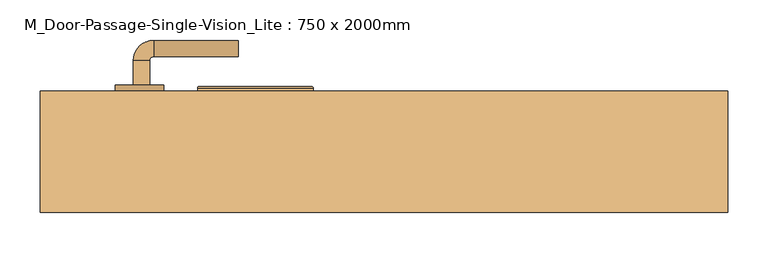
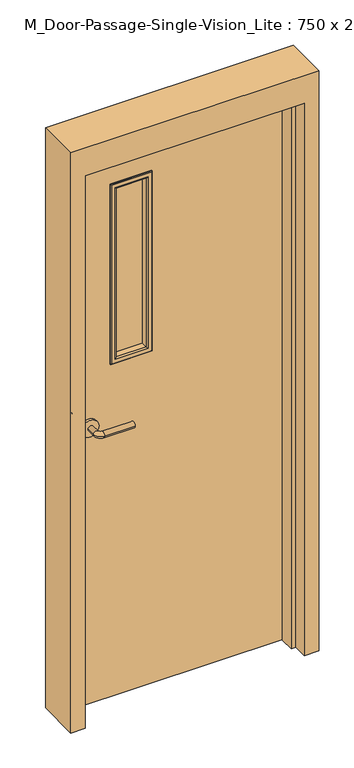
"""IFC4 building model written with IfcOpenShell, lengths in millimetres: door geometry, M_Door-Passage-Single-Vision_Lite : 750 x 2000mm."""

from ifc_helpers import new_model, si_unit, point, frame, frame_2d, origin, place, context, project, spatial, polyline, circle_curve, ellipse_curve, trimmed, segment, composite_curve, outline, extrude, faceted_brep, source, transform, mapped, element, save
from ifc_brep_helpers import plane_surface, cylinder_surface, revolved_surface, advanced_brep


def m_door_passage_single_vision_lite_750_x_2000mm_4b244377(model_context):
    return source(origin(), model_context, "Body", "SolidModel", [
        advanced_brep(
        [(-309.990625, 3.35, 1000.0), (-289.990625, 3.35, 1000.0), (-289.990625, -26.65, 1000.0), (-309.990625, -26.65, 1000.0), (-284.990625, -31.65, 1000.0), (-284.990625, -51.65, 1000.0), (-179.990625, -51.65, 1000.0), (-179.990625, -31.65, 1000.0)],
        [
            (0, 1, circle_curve(frame((-299.990625, 3.35, 1000.0), z_axis=(0.0, 1.0, 0.0), x_axis=(1.0, 0.0, 0.0)), 10.0)),
            (1, 0, circle_curve(frame((-299.990625, 3.35, 1000.0), z_axis=(0.0, 1.0, 0.0), x_axis=(1.0, 0.0, 0.0)), 10.0)),
            (1, 2),
            (2, 3, circle_curve(frame((-299.990625, -26.65, 1000.0), z_axis=(0.0, 1.0, 0.0), x_axis=(1.0, 0.0, 0.0)), 10.0)),
            (3, 0),
            (3, 2, circle_curve(frame((-299.990625, -26.65, 1000.0), z_axis=(0.0, 1.0, 0.0), x_axis=(1.0, 0.0, 0.0)), 10.0)),
            (4, 5, circle_curve(frame((-284.990625, -41.65, 1000.0), z_axis=(-1.0, 0.0, 0.0), x_axis=(0.0, 1.0, 0.0)), 10.0)),
            (5, 3, circle_curve(frame((-284.990625, -26.65, 1000.0), z_axis=(0.0, 0.0, -1.0), x_axis=(-1.0, 0.0, 0.0)), 25.0)),
            (2, 4, circle_curve(frame((-284.990625, -26.65, 1000.0), z_axis=(0.0, 0.0, 1.0), x_axis=(-1.0, 0.0, 0.0)), 5.0)),
            (5, 4, circle_curve(frame((-284.990625, -41.65, 1000.0), z_axis=(-1.0, 0.0, 0.0), x_axis=(0.0, 1.0, 0.0)), 10.0)),
            (6, 7, circle_curve(frame((-179.990625, -41.65, 1000.0), z_axis=(1.0, 0.0, 0.0), x_axis=(0.0, 1.0, 0.0)), 10.0)),
            (7, 6, circle_curve(frame((-179.990625, -41.65, 1000.0), z_axis=(1.0, 0.0, 0.0), x_axis=(0.0, 1.0, 0.0)), 10.0)),
            (4, 7),
            (6, 5),
        ],
        [
            plane_surface(frame((-299.990625, 3.35, 1000.0), z_axis=(0.0, 1.0, 0.0), x_axis=(0.0, 0.0, 1.0))),
            cylinder_surface(frame((-299.990625, 3.35, 1000.0), z_axis=(0.0, 1.0, 0.0), x_axis=(1.0, 0.0, 0.0)), 10.0),
            revolved_surface(trimmed(ellipse_curve(frame((-299.990625, -26.65, 1000.0), z_axis=(0.0, -1.0, 0.0), x_axis=(1.0, 0.0, 0.0)), 10.0, 10.0), [point((-309.990625, -26.65, 1000.0))], [point((-289.990625, -26.65, 1000.0))], True, "CARTESIAN"), (-284.990625, -26.65, 1000.0), (0.0, 0.0, -1.0)),
            revolved_surface(trimmed(ellipse_curve(frame((-299.990625, -26.65, 1000.0), z_axis=(0.0, -1.0, 0.0), x_axis=(1.0, 0.0, 0.0)), 10.0, 10.0), [point((-289.990625, -26.65, 1000.0))], [point((-309.990625, -26.65, 1000.0))], True, "CARTESIAN"), (-284.990625, -26.65, 1000.0), (0.0, 0.0, -1.0)),
            plane_surface(frame((-179.990625, -41.65, 1000.0), z_axis=(1.0, 0.0, 0.0), x_axis=(0.0, 0.0, 1.0))),
            cylinder_surface(frame((-284.990625, -41.65, 1000.0), z_axis=(-1.0, 0.0, 0.0), x_axis=(0.0, 1.0, 0.0)), 10.0),
        ],
        [
            (0, [[1, 2]]),
            (1, [[3, 4, 5, -2]]),
            (1, [[-5, 6, -3, -1]]),
            (2, [[7, 8, -4, 9]]),
            (3, [[10, -9, -6, -8]]),
            (4, [[11, 12]]),
            (5, [[13, -11, 14, -7]]),
            (5, [[-14, -12, -13, -10]]),
        ],
    ),
        extrude(outline(composite_curve([segment(trimmed(circle_curve(frame_2d((1000.0, -302.490625)), 30.0), [point((1000.0, -332.490625))], [point((1000.0, -272.490625))], False, "CARTESIAN"), True, "CONTINUOUS"), segment(trimmed(circle_curve(frame_2d((1000.0, -302.490625)), 30.0), [point((1000.0, -272.490625))], [point((1000.0, -332.490625))], False, "CARTESIAN"), True, "CONTINUOUS")], self_intersect=False)), frame((0.0, 3.35, 0.0), z_axis=(0.0, 1.0, 0.0), x_axis=(0.0, 0.0, 1.0)), (0.0, 0.0, 1.0), 8.0),
        advanced_brep(
        [(-309.990625, 64.35, 1000.0), (-289.990625, 64.35, 1000.0), (-309.990625, 94.35, 1000.0), (-289.990625, 94.35, 1000.0), (-284.990625, 99.35, 1000.0), (-284.990625, 119.35, 1000.0), (-179.990625, 119.35, 1000.0), (-179.990625, 99.35, 1000.0)],
        [
            (0, 1, circle_curve(frame((-299.990625, 64.35, 1000.0), z_axis=(0.0, -1.0, 0.0), x_axis=(1.0, 0.0, 0.0)), 10.0)),
            (1, 0, circle_curve(frame((-299.990625, 64.35, 1000.0), z_axis=(0.0, -1.0, 0.0), x_axis=(1.0, 0.0, 0.0)), 10.0)),
            (0, 2),
            (2, 3, circle_curve(frame((-299.990625, 94.35, 1000.0), z_axis=(0.0, -1.0, 0.0), x_axis=(1.0, 0.0, 0.0)), 10.0)),
            (3, 1),
            (3, 2, circle_curve(frame((-299.990625, 94.35, 1000.0), z_axis=(0.0, -1.0, 0.0), x_axis=(1.0, 0.0, 0.0)), 10.0)),
            (4, 3, circle_curve(frame((-284.990625, 94.35, 1000.0), z_axis=(0.0, 0.0, 1.0), x_axis=(-1.0, 0.0, 0.0)), 5.0)),
            (2, 5, circle_curve(frame((-284.990625, 94.35, 1000.0), z_axis=(0.0, 0.0, -1.0), x_axis=(-1.0, 0.0, 0.0)), 25.0)),
            (5, 4, circle_curve(frame((-284.990625, 109.35, 1000.0), z_axis=(-1.0, 0.0, 0.0), x_axis=(0.0, -1.0, 0.0)), 10.0)),
            (4, 5, circle_curve(frame((-284.990625, 109.35, 1000.0), z_axis=(-1.0, 0.0, 0.0), x_axis=(0.0, -1.0, 0.0)), 10.0)),
            (6, 7, circle_curve(frame((-179.990625, 109.35, 1000.0), z_axis=(1.0, 0.0, 0.0), x_axis=(0.0, -1.0, 0.0)), 10.0)),
            (7, 6, circle_curve(frame((-179.990625, 109.35, 1000.0), z_axis=(1.0, 0.0, 0.0), x_axis=(0.0, -1.0, 0.0)), 10.0)),
            (5, 6),
            (7, 4),
        ],
        [
            plane_surface(frame((-299.990625, 64.35, 1000.0), z_axis=(0.0, -1.0, 0.0), x_axis=(0.0, 0.0, 1.0))),
            cylinder_surface(frame((-299.990625, 64.35, 1000.0), z_axis=(0.0, -1.0, 0.0), x_axis=(1.0, 0.0, 0.0)), 10.0),
            revolved_surface(trimmed(ellipse_curve(frame((-299.990625, 94.35, 1000.0), z_axis=(0.0, -1.0, 0.0), x_axis=(1.0, 0.0, 0.0)), 10.0, 10.0), [point((-309.990625, 94.35, 1000.0))], [point((-289.990625, 94.35, 1000.0))], True, "CARTESIAN"), (-284.990625, 94.35, 1000.0), (0.0, 0.0, -1.0)),
            revolved_surface(trimmed(ellipse_curve(frame((-299.990625, 94.35, 1000.0), z_axis=(0.0, -1.0, 0.0), x_axis=(1.0, 0.0, 0.0)), 10.0, 10.0), [point((-289.990625, 94.35, 1000.0))], [point((-309.990625, 94.35, 1000.0))], True, "CARTESIAN"), (-284.990625, 94.35, 1000.0), (0.0, 0.0, -1.0)),
            plane_surface(frame((-179.990625, 109.35, 1000.0), z_axis=(1.0, 0.0, 0.0), x_axis=(0.0, 0.0, 1.0))),
            cylinder_surface(frame((-284.990625, 109.35, 1000.0), z_axis=(-1.0, 0.0, 0.0), x_axis=(0.0, -1.0, 0.0)), 10.0),
        ],
        [
            (0, [[1, 2]]),
            (1, [[-1, 3, 4, 5]]),
            (1, [[-2, -5, 6, -3]]),
            (2, [[7, -4, 8, 9]]),
            (3, [[-8, -6, -7, 10]]),
            (4, [[11, 12]]),
            (5, [[-9, 13, -12, 14]]),
            (5, [[-10, -14, -11, -13]]),
        ],
    ),
        extrude(outline(composite_curve([segment(trimmed(circle_curve(frame_2d((1000.0, -302.490625)), 30.0), [point((1000.0, -332.490625))], [point((1000.0, -272.490625))], False, "CARTESIAN"), True, "CONTINUOUS"), segment(trimmed(circle_curve(frame_2d((1000.0, -302.490625)), 30.0), [point((1000.0, -272.490625))], [point((1000.0, -332.490625))], False, "CARTESIAN"), True, "CONTINUOUS")], self_intersect=False)), frame((0.0, 56.35, 0.0), z_axis=(0.0, 1.0, 0.0), x_axis=(0.0, 0.0, 1.0)), (0.0, 0.0, 1.0), 8.0),
        extrude(outline(polyline([(2000.0, -375.0), (0.0, -375.0), (0.0, 375.0), (2000.0, 375.0), (2000.0, -375.0)]), holes=[polyline([(1847.6, -222.6), (1847.6, -95.6), (1212.6, -95.6), (1212.6, -222.6), (1847.6, -222.6)])]), frame((0.0, 11.35, 0.0), z_axis=(0.0, 1.0, 0.0), x_axis=(0.0, 0.0, 1.0)), (0.0, 0.0, 1.0), 45.0),
        faceted_brep([(375.0, 6.5875, 0.0), (375.0, 56.35, 0.0), (425.0, 56.35, 0.0), (425.0, -93.65, 0.0), (375.0, -93.65, 0.0), (375.0, -44.4375, 0.0), (359.125, -44.4375, 0.0), (359.125, 6.5875, 0.0), (375.0, 6.5875, 2000.0), (375.0, 56.35, 2000.0), (-375.0, 56.35, 2000.0), (-375.0, 56.35, 0.0), (-425.0, 56.35, 0.0), (-425.0, 56.35, 2100.0), (425.0, 56.35, 2100.0), (425.0, -93.65, 2100.0), (-425.0, -93.65, 2100.0), (-425.0, -93.65, 0.0), (-375.0, -93.65, 0.0), (-375.0, -93.65, 2000.0), (375.0, -93.65, 2000.0), (375.0, -44.4375, 2000.0), (-375.0, -44.4375, 2000.0), (-375.0, -44.4375, 0.0), (-359.125, -44.4375, 0.0), (-359.125, -44.4375, 1984.125), (359.125, -44.4375, 1984.125), (359.125, 6.5875, 1984.125), (-359.125, 6.5875, 1984.125), (-359.125, 6.5875, 0.0), (-375.0, 6.5875, 0.0), (-375.0, 6.5875, 2000.0)], [[[0, 1, 2, 3, 4, 5, 6, 7]], [[1, 0, 8, 9]], [[2, 1, 9, 10, 11, 12, 13, 14]], [[3, 2, 14, 15]], [[4, 3, 15, 16, 17, 18, 19, 20]], [[5, 4, 20, 21]], [[6, 5, 21, 22, 23, 24, 25, 26]], [[7, 6, 26, 27]], [[0, 7, 27, 28, 29, 30, 31, 8]], [[9, 8, 31, 10]], [[20, 19, 22, 21]], [[26, 25, 28, 27]], [[12, 11, 30, 29, 24, 23, 18, 17]], [[11, 10, 31, 30]], [[13, 12, 17, 16]], [[19, 18, 23, 22]], [[25, 24, 29, 28]], [[15, 14, 13, 16]]]),
        extrude(outline(polyline([(-95.6, 31.35), (-222.6, 31.35), (-222.6, 36.35), (-95.6, 36.35), (-95.6, 31.35)])), frame((0.0, 0.0, 1212.6), z_axis=(0.0, 0.0, 1.0), x_axis=(1.0, 0.0, 0.0)), (0.0, 0.0, 1.0), 635.0),
        advanced_brep(
        [(-222.6, 36.35, 1847.6), (-222.6, 56.35, 1847.6), (-222.6, 56.35, 1212.6), (-222.6, 36.35, 1212.6), (-210.6, 57.35, 1835.6), (-210.6, 36.35, 1835.6), (-210.6, 36.35, 1224.6), (-210.6, 57.35, 1224.6), (-215.6, 62.35, 1840.6), (-215.6, 62.35, 1219.6), (-230.6, 60.35, 1855.6), (-228.6, 62.35, 1853.6), (-228.6, 62.35, 1206.6), (-230.6, 60.35, 1204.6), (-230.6, 56.35, 1855.6), (-230.6, 56.35, 1204.6), (-95.6, 56.35, 1212.6), (-95.6, 36.35, 1212.6), (-107.6, 36.35, 1224.6), (-107.6, 57.35, 1224.6), (-102.6, 62.35, 1219.6), (-89.6, 62.35, 1206.6), (-87.6, 60.35, 1204.6), (-87.6, 56.35, 1204.6), (-95.6, 56.35, 1847.6), (-95.6, 36.35, 1847.6), (-107.6, 36.35, 1835.6), (-107.6, 57.35, 1835.6), (-102.6, 62.35, 1840.6), (-89.6, 62.35, 1853.6), (-87.6, 60.35, 1855.6), (-87.6, 56.35, 1855.6)],
        [
            (0, 1),
            (1, 2),
            (2, 3),
            (3, 0),
            (4, 5),
            (5, 6),
            (6, 7),
            (7, 4),
            (8, 4, ellipse_curve(frame((-215.6, 57.35, 1840.6), z_axis=(-0.7071067811865475, 0.0, -0.7071067811865475), x_axis=(-0.7071067811865474, 0.0, 0.7071067811865476)), 7.0710678, 5.0)),
            (7, 9, ellipse_curve(frame((-215.6, 57.35, 1219.6), z_axis=(-0.7071067811865475, 0.0, 0.7071067811865475), x_axis=(0.7071067811865474, 0.0, 0.7071067811865476)), 7.0710678, 5.0)),
            (9, 8),
            (10, 11, ellipse_curve(frame((-228.6, 60.35, 1853.6), z_axis=(-0.7071067811865475, 0.0, -0.7071067811865475), x_axis=(-0.7071067811865474, 0.0, 0.7071067811865476)), 2.8284271, 2.0)),
            (11, 12),
            (12, 13, ellipse_curve(frame((-228.6, 60.35, 1206.6), z_axis=(-0.7071067811865475, 0.0, 0.7071067811865475), x_axis=(0.7071067811865474, 0.0, 0.7071067811865476)), 2.8284271, 2.0)),
            (13, 10),
            (14, 10),
            (13, 15),
            (15, 14),
            (2, 16),
            (16, 17),
            (17, 3),
            (6, 18),
            (18, 19),
            (19, 7),
            (19, 20, ellipse_curve(frame((-102.6, 57.35, 1219.6), z_axis=(-0.7071067811865475, 0.0, -0.7071067811865475), x_axis=(-0.7071067811865476, 0.0, 0.7071067811865474)), 7.0710678, 5.0)),
            (20, 9),
            (12, 21),
            (21, 22, ellipse_curve(frame((-89.6, 60.35, 1206.6), z_axis=(-0.7071067811865475, 0.0, -0.7071067811865475), x_axis=(-0.7071067811865476, 0.0, 0.7071067811865474)), 2.8284271, 2.0)),
            (22, 13),
            (22, 23),
            (23, 15),
            (16, 24),
            (24, 25),
            (25, 17),
            (18, 26),
            (26, 27),
            (27, 19),
            (27, 28, ellipse_curve(frame((-102.6, 57.35, 1840.6), z_axis=(0.7071067811865475, 0.0, -0.7071067811865475), x_axis=(-0.7071067811865474, 0.0, -0.7071067811865476)), 7.0710678, 5.0)),
            (28, 20),
            (21, 29),
            (29, 30, ellipse_curve(frame((-89.6, 60.35, 1853.6), z_axis=(0.7071067811865475, 0.0, -0.7071067811865475), x_axis=(-0.7071067811865474, 0.0, -0.7071067811865476)), 2.8284271, 2.0)),
            (30, 22),
            (30, 31),
            (31, 23),
            (31, 14),
            (1, 24),
            (0, 25),
            (5, 26),
            (4, 27),
            (8, 28),
            (11, 29),
            (10, 30),
        ],
        [
            plane_surface(frame((-222.6, 56.35, 1847.6), z_axis=(-1.0, 0.0, 0.0), x_axis=(0.0, 0.0, -1.0))),
            plane_surface(frame((-210.6, 36.35, 1835.6), z_axis=(1.0, 0.0, 0.0), x_axis=(0.0, 0.0, -1.0))),
            cylinder_surface(frame((-215.6, 57.35, 1847.6), z_axis=(0.0, 0.0, 1.0), x_axis=(-1.0, 0.0, 0.0)), 5.0),
            cylinder_surface(frame((-228.6, 60.35, 1847.6), z_axis=(0.0, 0.0, 1.0), x_axis=(-1.0, 0.0, 0.0)), 2.0),
            plane_surface(frame((-230.6, 60.35, 1855.6), z_axis=(-1.0, 0.0, 0.0), x_axis=(0.0, 0.0, -1.0))),
            plane_surface(frame((-222.6, 56.35, 1212.6), z_axis=(0.0, 0.0, -1.0), x_axis=(1.0, 0.0, 0.0))),
            plane_surface(frame((-210.6, 36.35, 1224.6), z_axis=(0.0, 0.0, 1.0), x_axis=(1.0, 0.0, 0.0))),
            cylinder_surface(frame((-222.6, 57.35, 1219.6), z_axis=(-1.0, 0.0, 0.0), x_axis=(0.0, 0.0, -1.0)), 5.0),
            cylinder_surface(frame((-222.6, 60.35, 1206.6), z_axis=(-1.0, 0.0, 0.0), x_axis=(0.0, 0.0, -1.0)), 2.0),
            plane_surface(frame((-230.6, 60.35, 1204.6), z_axis=(0.0, 0.0, -1.0), x_axis=(1.0, 0.0, 0.0))),
            plane_surface(frame((-95.6, 56.35, 1212.6), z_axis=(1.0, 0.0, 0.0), x_axis=(0.0, 0.0, 1.0))),
            plane_surface(frame((-107.6, 36.35, 1224.6), z_axis=(-1.0, 0.0, 0.0), x_axis=(0.0, 0.0, 1.0))),
            cylinder_surface(frame((-102.6, 57.35, 1212.6), z_axis=(0.0, 0.0, -1.0), x_axis=(1.0, 0.0, 0.0)), 5.0),
            cylinder_surface(frame((-89.6, 60.35, 1212.6), z_axis=(0.0, 0.0, -1.0), x_axis=(1.0, 0.0, 0.0)), 2.0),
            plane_surface(frame((-87.6, 60.35, 1204.6), z_axis=(1.0, 0.0, 0.0), x_axis=(0.0, 0.0, 1.0))),
            plane_surface(frame((-87.6, 56.35, 1855.6), z_axis=(0.0, -1.0, 0.0), x_axis=(-1.0, 0.0, 0.0))),
            plane_surface(frame((-95.6, 56.35, 1847.6), z_axis=(0.0, 0.0, 1.0), x_axis=(-1.0, 0.0, 0.0))),
            plane_surface(frame((-95.6, 36.35, 1847.6), z_axis=(0.0, -1.0, 0.0), x_axis=(-1.0, 0.0, 0.0))),
            plane_surface(frame((-107.6, 36.35, 1835.6), z_axis=(0.0, 0.0, -1.0), x_axis=(-1.0, 0.0, 0.0))),
            cylinder_surface(frame((-95.6, 57.35, 1840.6), z_axis=(1.0, 0.0, 0.0), x_axis=(0.0, 0.0, 1.0)), 5.0),
            plane_surface(frame((-102.6, 62.35, 1840.6), z_axis=(0.0, 1.0, 0.0), x_axis=(-1.0, 0.0, 0.0))),
            cylinder_surface(frame((-95.6, 60.35, 1853.6), z_axis=(1.0, 0.0, 0.0), x_axis=(0.0, 0.0, 1.0)), 2.0),
            plane_surface(frame((-87.6, 60.35, 1855.6), z_axis=(0.0, 0.0, 1.0), x_axis=(-1.0, 0.0, 0.0))),
        ],
        [
            (0, [[1, 2, 3, 4]]),
            (1, [[5, 6, 7, 8]]),
            (2, [[9, -8, 10, 11]]),
            (3, [[12, 13, 14, 15]]),
            (4, [[16, -15, 17, 18]]),
            (5, [[-3, 19, 20, 21]]),
            (6, [[-7, 22, 23, 24]]),
            (7, [[-10, -24, 25, 26]]),
            (8, [[-14, 27, 28, 29]]),
            (9, [[-17, -29, 30, 31]]),
            (10, [[-20, 32, 33, 34]]),
            (11, [[-23, 35, 36, 37]]),
            (12, [[-25, -37, 38, 39]]),
            (13, [[-28, 40, 41, 42]]),
            (14, [[-30, -42, 43, 44]]),
            (15, [[-31, -44, 45, -18], [46, -32, -19, -2]]),
            (16, [[-33, -46, -1, 47]]),
            (17, [[-21, -34, -47, -4], [48, -35, -22, -6]]),
            (18, [[-36, -48, -5, 49]]),
            (19, [[-38, -49, -9, 50]]),
            (20, [[51, -40, -27, -13], [-26, -39, -50, -11]]),
            (21, [[-41, -51, -12, 52]]),
            (22, [[-43, -52, -16, -45]]),
        ],
    ),
        advanced_brep(
        [(-222.6, 31.35, 1212.6), (-222.6, 11.35, 1212.6), (-222.6, 11.35, 1847.6), (-222.6, 31.35, 1847.6), (-210.6, 10.35, 1224.6), (-210.6, 31.35, 1224.6), (-210.6, 31.35, 1835.6), (-210.6, 10.35, 1835.6), (-215.6, 5.35, 1219.6), (-215.6, 5.35, 1840.6), (-230.6, 7.35, 1204.6), (-228.6, 5.35, 1206.6), (-228.6, 5.35, 1853.6), (-230.6, 7.35, 1855.6), (-230.6, 11.35, 1204.6), (-230.6, 11.35, 1855.6), (-95.6, 11.35, 1847.6), (-95.6, 31.35, 1847.6), (-107.6, 31.35, 1835.6), (-107.6, 10.35, 1835.6), (-102.6, 5.35, 1840.6), (-89.6, 5.35, 1853.6), (-87.6, 7.35, 1855.6), (-87.6, 11.35, 1855.6), (-95.6, 11.35, 1212.6), (-95.6, 31.35, 1212.6), (-107.6, 31.35, 1224.6), (-107.6, 10.35, 1224.6), (-102.6, 5.35, 1219.6), (-89.6, 5.35, 1206.6), (-87.6, 7.35, 1204.6), (-87.6, 11.35, 1204.6)],
        [
            (0, 1),
            (1, 2),
            (2, 3),
            (3, 0),
            (4, 5),
            (5, 6),
            (6, 7),
            (7, 4),
            (8, 4, ellipse_curve(frame((-215.6, 10.35, 1219.6), z_axis=(-0.7071067811865475, 0.0, 0.7071067811865475), x_axis=(-0.7071067811865474, 0.0, -0.7071067811865476)), 7.0710678, 5.0)),
            (7, 9, ellipse_curve(frame((-215.6, 10.35, 1840.6), z_axis=(-0.7071067811865475, 0.0, -0.7071067811865475), x_axis=(0.7071067811865474, 0.0, -0.7071067811865476)), 7.0710678, 5.0)),
            (9, 8),
            (10, 11, ellipse_curve(frame((-228.6, 7.35, 1206.6), z_axis=(-0.7071067811865475, 0.0, 0.7071067811865475), x_axis=(-0.7071067811865474, 0.0, -0.7071067811865476)), 2.8284271, 2.0)),
            (11, 12),
            (12, 13, ellipse_curve(frame((-228.6, 7.35, 1853.6), z_axis=(-0.7071067811865475, 0.0, -0.7071067811865475), x_axis=(0.7071067811865474, 0.0, -0.7071067811865476)), 2.8284271, 2.0)),
            (13, 10),
            (14, 10),
            (13, 15),
            (15, 14),
            (2, 16),
            (16, 17),
            (17, 3),
            (6, 18),
            (18, 19),
            (19, 7),
            (19, 20, ellipse_curve(frame((-102.6, 10.35, 1840.6), z_axis=(-0.7071067811865475, 0.0, 0.7071067811865475), x_axis=(-0.7071067811865476, 0.0, -0.7071067811865474)), 7.0710678, 5.0)),
            (20, 9),
            (12, 21),
            (21, 22, ellipse_curve(frame((-89.6, 7.35, 1853.6), z_axis=(-0.7071067811865475, 0.0, 0.7071067811865475), x_axis=(-0.7071067811865476, 0.0, -0.7071067811865474)), 2.8284271, 2.0)),
            (22, 13),
            (22, 23),
            (23, 15),
            (16, 24),
            (24, 25),
            (25, 17),
            (18, 26),
            (26, 27),
            (27, 19),
            (27, 28, ellipse_curve(frame((-102.6, 10.35, 1219.6), z_axis=(0.7071067811865475, 0.0, 0.7071067811865475), x_axis=(-0.7071067811865474, 0.0, 0.7071067811865476)), 7.0710678, 5.0)),
            (28, 20),
            (21, 29),
            (29, 30, ellipse_curve(frame((-89.6, 7.35, 1206.6), z_axis=(0.7071067811865475, 0.0, 0.7071067811865475), x_axis=(-0.7071067811865474, 0.0, 0.7071067811865476)), 2.8284271, 2.0)),
            (30, 22),
            (30, 31),
            (31, 23),
            (31, 14),
            (1, 24),
            (0, 25),
            (5, 26),
            (4, 27),
            (8, 28),
            (11, 29),
            (10, 30),
        ],
        [
            plane_surface(frame((-222.6, 11.35, 1212.6), z_axis=(-1.0, 0.0, 0.0), x_axis=(0.0, 0.0, 1.0))),
            plane_surface(frame((-210.6, 31.35, 1224.6), z_axis=(1.0, 0.0, 0.0), x_axis=(0.0, 0.0, 1.0))),
            cylinder_surface(frame((-215.6, 10.35, 1212.6), z_axis=(0.0, 0.0, -1.0), x_axis=(-1.0, 0.0, 0.0)), 5.0),
            cylinder_surface(frame((-228.6, 7.35, 1212.6), z_axis=(0.0, 0.0, -1.0), x_axis=(-1.0, 0.0, 0.0)), 2.0),
            plane_surface(frame((-230.6, 7.35, 1204.6), z_axis=(-1.0, 0.0, 0.0), x_axis=(0.0, 0.0, 1.0))),
            plane_surface(frame((-222.6, 11.35, 1847.6), z_axis=(0.0, 0.0, 1.0), x_axis=(1.0, 0.0, 0.0))),
            plane_surface(frame((-210.6, 31.35, 1835.6), z_axis=(0.0, 0.0, -1.0), x_axis=(1.0, 0.0, 0.0))),
            cylinder_surface(frame((-222.6, 10.35, 1840.6), z_axis=(-1.0, 0.0, 0.0), x_axis=(0.0, 0.0, 1.0)), 5.0),
            cylinder_surface(frame((-222.6, 7.35, 1853.6), z_axis=(-1.0, 0.0, 0.0), x_axis=(0.0, 0.0, 1.0)), 2.0),
            plane_surface(frame((-230.6, 7.35, 1855.6), z_axis=(0.0, 0.0, 1.0), x_axis=(1.0, 0.0, 0.0))),
            plane_surface(frame((-95.6, 11.35, 1847.6), z_axis=(1.0, 0.0, 0.0), x_axis=(0.0, 0.0, -1.0))),
            plane_surface(frame((-107.6, 31.35, 1835.6), z_axis=(-1.0, 0.0, 0.0), x_axis=(0.0, 0.0, -1.0))),
            cylinder_surface(frame((-102.6, 10.35, 1847.6), z_axis=(0.0, 0.0, 1.0), x_axis=(1.0, 0.0, 0.0)), 5.0),
            cylinder_surface(frame((-89.6, 7.35, 1847.6), z_axis=(0.0, 0.0, 1.0), x_axis=(1.0, 0.0, 0.0)), 2.0),
            plane_surface(frame((-87.6, 7.35, 1855.6), z_axis=(1.0, 0.0, 0.0), x_axis=(0.0, 0.0, -1.0))),
            plane_surface(frame((-87.6, 11.35, 1204.6), z_axis=(0.0, 1.0, 0.0), x_axis=(-1.0, 0.0, 0.0))),
            plane_surface(frame((-95.6, 11.35, 1212.6), z_axis=(0.0, 0.0, -1.0), x_axis=(-1.0, 0.0, 0.0))),
            plane_surface(frame((-95.6, 31.35, 1212.6), z_axis=(0.0, 1.0, 0.0), x_axis=(-1.0, 0.0, 0.0))),
            plane_surface(frame((-107.6, 31.35, 1224.6), z_axis=(0.0, 0.0, 1.0), x_axis=(-1.0, 0.0, 0.0))),
            cylinder_surface(frame((-95.6, 10.35, 1219.6), z_axis=(1.0, 0.0, 0.0), x_axis=(0.0, 0.0, -1.0)), 5.0),
            plane_surface(frame((-102.6, 5.35, 1219.6), z_axis=(0.0, -1.0, 0.0), x_axis=(-1.0, 0.0, 0.0))),
            cylinder_surface(frame((-95.6, 7.35, 1206.6), z_axis=(1.0, 0.0, 0.0), x_axis=(0.0, 0.0, -1.0)), 2.0),
            plane_surface(frame((-87.6, 7.35, 1204.6), z_axis=(0.0, 0.0, -1.0), x_axis=(-1.0, 0.0, 0.0))),
        ],
        [
            (0, [[1, 2, 3, 4]]),
            (1, [[5, 6, 7, 8]]),
            (2, [[9, -8, 10, 11]]),
            (3, [[12, 13, 14, 15]]),
            (4, [[16, -15, 17, 18]]),
            (5, [[-3, 19, 20, 21]]),
            (6, [[-7, 22, 23, 24]]),
            (7, [[-10, -24, 25, 26]]),
            (8, [[-14, 27, 28, 29]]),
            (9, [[-17, -29, 30, 31]]),
            (10, [[-20, 32, 33, 34]]),
            (11, [[-23, 35, 36, 37]]),
            (12, [[-25, -37, 38, 39]]),
            (13, [[-28, 40, 41, 42]]),
            (14, [[-30, -42, 43, 44]]),
            (15, [[-31, -44, 45, -18], [46, -32, -19, -2]]),
            (16, [[-33, -46, -1, 47]]),
            (17, [[-21, -34, -47, -4], [48, -35, -22, -6]]),
            (18, [[-36, -48, -5, 49]]),
            (19, [[-38, -49, -9, 50]]),
            (20, [[51, -40, -27, -13], [-26, -39, -50, -11]]),
            (21, [[-41, -51, -12, 52]]),
            (22, [[-43, -52, -16, -45]]),
        ],
    ),
    ])


if __name__ == "__main__":
    model = new_model("IFC4")
    model_context = context("Model", 3, world=origin())
    ifc_project = project(units=[si_unit("LENGTHUNIT", "METRE", prefix="MILLI")], contexts=[model_context])
    site = spatial("IfcSite", under=ifc_project)
    building = spatial("IfcBuilding", under=site)
    placement = place(None, origin())
    m_door_passage_single_vision_lite_750_x_2000mm_shape = m_door_passage_single_vision_lite_750_x_2000mm_4b244377(model_context)
    element("IfcDoor", 1, ObjectType="M_Door-Passage-Single-Vision_Lite : 750 x 2000mm", at=placement, inside=building, context=model_context, shape_type="MappedRepresentation", body=[
        mapped(m_door_passage_single_vision_lite_750_x_2000mm_shape, transform((0.0, 0.0, 0.0), x_axis=(1.0, 0.0, 0.0), y_axis=(0.0, 1.0, 0.0), z_axis=(0.0, 0.0, 1.0))),
    ])
    save(model, "model.ifc")

# Revit data of these elements
# Project information
#   Organization Name = "Organization Name"
#   Organization Description = "Organization Description"
#   Building Name = "Building Name"
#   Project Issue Date = "Issue Date"
#   Project Status = "Project Status"
#   Client Name = "Client Name"
#   Project Address = "Enter address here\nAddress Line 2"
#   Project Name = "Project Name"
#   Project Number = "Project Number"
# Type "M_Door-Passage-Single-Vision_Lite : 750 x 2000mm"
#   Type Mark = "42"
#   Analytic Construction = "Wooden"
#   Thickness = 45 mm
#   Thermal Resistance (R) = 0.455703 (m²·K)/W
#   Swing Angle [instance default] = 90.00°
#   Strike Height = 1000 mm
#   Rough Width [instance default] = 850 mm
#   Rough Height [instance default] = 2100 mm
#   MFOpeningHeight [instance default] = 100 mm
#   MFOpeningWidth [instance default] = 100 mm
#   Inset Calculate [instance default] = 105 mm
#   Masonry Inset [instance default] = 25 mm
#   Height = 2000 mm
#   Width = 750 mm
#   Heat Transfer Coefficient (U) = 2.19465 W/(m²·K)
#   Masonry Frame Depth = 150 mm
#   Masonry Frame [instance default] = yes
#   Function = 1
#   Dry Wall Frame [instance default] = no
#   Panel Material = Wood - Birch
#   Glazing = Glass
#   Glass Stop Material = Metal - Paint Finish - Grey
#   Frame Material = Metal - Paint Finish - Grey
#   Door Handle Material = Aluminum
#   Visual Light Transmittance = 0
#   Solar Heat Gain Coefficient = 0
#   Wall Closure = (empty or 0)
# Element 1 (IfcDoor, "M_Door-Passage-Single-Vision_Lite : 750 x 2000mm")
#   Materials on its faces: "Metal - Paint Finish - Grey", "Aluminum", "Wood - Birch", "Glass"
# Materials
#   "Wood - Birch": class "Wood", colour RGB 173 132 96, transparency 0, Cost = 0
#   "Glass": class "Glass", colour RGB 245 245 243, transparency 1, Description = "Soda Lime Glass", Cost = 0
#   "Metal - Paint Finish - Grey": class "Paint", colour RGB 178 178 178, transparency 0, Cost = 0
#   "Aluminum": class "Metal", colour RGB 244 245 246, transparency 0, Description = "Aluminum 6061", Cost = 0
